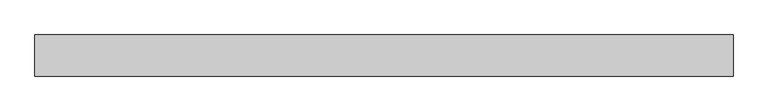
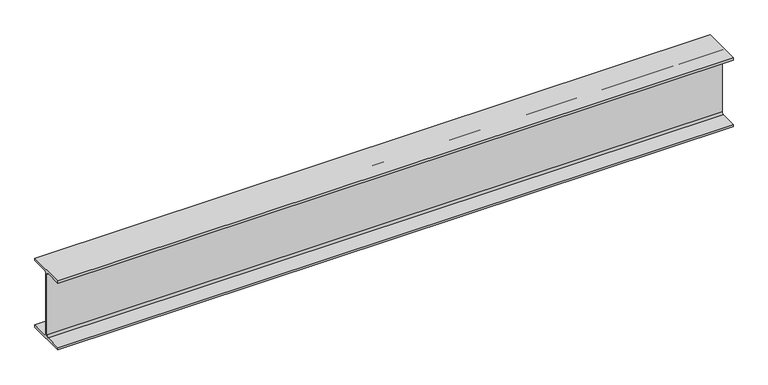
"""IFC4 building model written with IfcOpenShell, lengths in millimetres: beam geometry, Steel Beam_H-KSD3502 : H_SB_ASB_H-200x200x8x12."""

import ifcopenshell
import ifcopenshell.guid

model = None  # the IFC model being written
_history = None  # IfcOwnerHistory: only IFC2X3 demands one
_inside = {}  # id of a spatial element -> (the spatial element, [elements in it])
_under = {}  # id of a project, library or spatial element -> (it, [spatial elements below it])
_declared = {}  # id of a project -> (the project, [libraries it declares])
_typed = {}  # id of a type object -> (the type object, [elements of that type])
_made_of = {}  # id of a material, layer set ... -> (it, [elements and type objects made of it])


def new_model(schema):
    """Start an empty IFC model of exactly this schema.

    Asked for "IFC4X3", IfcOpenShell would pick the latest addendum, in which some entities
    have other attributes; the version numbers below select the first issue.
    IFC2X3 requires an IfcOwnerHistory on every rooted entity: one is made here for all.
    """
    global model, _history
    if schema == "IFC4X3":
        model = ifcopenshell.file(schema_version=(4, 3, 0, 0))
    else:
        model = ifcopenshell.file(schema=schema)
    _inside.clear()
    _under.clear()
    _declared.clear()
    _typed.clear()
    _made_of.clear()
    _history = None
    if model.schema == "IFC2X3":
        org = make("IfcOrganization", Name="unknown")
        user = make(
            "IfcPersonAndOrganization",
            ThePerson=make("IfcPerson", FamilyName="unknown"),
            TheOrganization=org,
        )
        app = make(
            "IfcApplication",
            ApplicationDeveloper=org,
            Version="unknown",
            ApplicationFullName="unknown",
            ApplicationIdentifier="unknown",
        )
        _history = make(
            "IfcOwnerHistory",
            OwningUser=user,
            OwningApplication=app,
            ChangeAction="ADDED",
            CreationDate=0,
        )
    return model


def make(cls, **values):
    """One entity of the class cls with the attributes given. An attribute that is None is left unset."""
    return model.create_entity(
        cls, **{name: value for name, value in values.items() if value is not None}
    )


def rooted(cls, **values):
    """An entity with a GlobalId (a new one), such as an element, a storey or a relation."""
    return make(cls, GlobalId=ifcopenshell.guid.new(), OwnerHistory=_history, **values)


def si_unit(unit_type, name, prefix=None):
    """IfcSIUnit, for example si_unit("LENGTHUNIT", "METRE", prefix="MILLI")."""
    return make("IfcSIUnit", UnitType=unit_type, Prefix=prefix, Name=name)


def assignment(units):
    """IfcUnitAssignment: the units of a project."""
    return None if units is None else make("IfcUnitAssignment", Units=units)


def point(xyz):
    """IfcCartesianPoint."""
    return None if xyz is None else make("IfcCartesianPoint", Coordinates=xyz)


def direction(xyz):
    """IfcDirection."""
    return None if xyz is None else make("IfcDirection", DirectionRatios=xyz)


def frame(location, z_axis=None, x_axis=None):
    """IfcAxis2Placement3D, a coordinate frame: its origin and axes. An axis left out is left unset."""
    return make(
        "IfcAxis2Placement3D",
        Location=point(location),
        Axis=direction(z_axis),
        RefDirection=direction(x_axis),
    )


def frame_2d(location, x_axis=None):
    """IfcAxis2Placement2D, a coordinate frame in the plane: its origin and x axis."""
    return make(
        "IfcAxis2Placement2D", Location=point(location), RefDirection=direction(x_axis)
    )


def origin():
    """The frame at (0, 0, 0) with its axes left unset."""
    return frame((0.0, 0.0, 0.0))


def place(relative_to, where):
    """IfcLocalPlacement: puts the frame where relative to a parent placement (None: the world)."""
    return make(
        "IfcLocalPlacement", PlacementRelTo=relative_to, RelativePlacement=where
    )


def context(
    kind, dimensions, precision=None, world=None, true_north=None, identifier=None
):
    """IfcGeometricRepresentationContext, for example the 3D "Model" context."""
    return make(
        "IfcGeometricRepresentationContext",
        ContextIdentifier=identifier,
        ContextType=kind,
        CoordinateSpaceDimension=dimensions,
        Precision=precision,
        WorldCoordinateSystem=world,
        TrueNorth=true_north,
    )


def project(units=None, contexts=None):
    """IfcProject with its units and contexts."""
    return rooted(
        "IfcProject",
        Name="project",
        RepresentationContexts=contexts,
        UnitsInContext=assignment(units),
    )


def spatial(cls, under=None, at=None, **own):
    """A site, building, storey or space (cls), placed at a placement, below another one or the project."""
    s = rooted(cls, ObjectPlacement=at, **own)
    if under is not None:
        _under.setdefault(under.id(), (under, []))[1].append(s)
    return s


def polyline(points):
    """IfcPolyline through the points."""
    return make("IfcPolyline", Points=[point(p) for p in points])


def circle_curve(where, radius):
    """IfcCircle in the frame where."""
    return make("IfcCircle", Position=where, Radius=radius)


def trimmed(basis, trim1, trim2, sense, master):
    """IfcTrimmedCurve: the piece of a basis curve between two trims."""
    return make(
        "IfcTrimmedCurve",
        BasisCurve=basis,
        Trim1=trim1,
        Trim2=trim2,
        SenseAgreement=sense,
        MasterRepresentation=master,
    )


def segment(curve, same_sense, transition):
    """IfcCompositeCurveSegment."""
    return make(
        "IfcCompositeCurveSegment",
        Transition=transition,
        SameSense=same_sense,
        ParentCurve=curve,
    )


def composite_curve(segments, self_intersect=None):
    """IfcCompositeCurve: segments joined end to end."""
    return make("IfcCompositeCurve", Segments=segments, SelfIntersect=self_intersect)


def outline(outer, holes=None, kind="AREA"):
    """IfcArbitraryClosedProfileDef: a profile drawn as a closed curve; with holes, ...WithVoids."""
    if holes is None:
        return make("IfcArbitraryClosedProfileDef", ProfileType=kind, OuterCurve=outer)
    return make(
        "IfcArbitraryProfileDefWithVoids",
        ProfileType=kind,
        OuterCurve=outer,
        InnerCurves=holes,
    )


def extrude(swept, where, along, depth):
    """IfcExtrudedAreaSolid: the profile swept, set in the frame where, extruded along a direction by depth."""
    return make(
        "IfcExtrudedAreaSolid",
        SweptArea=swept,
        Position=where,
        ExtrudedDirection=direction(along),
        Depth=depth,
    )


def shape(context_of_items, identifier, shape_type, items):
    """IfcShapeRepresentation: the items that make up one representation, for example the "Body"."""
    return make(
        "IfcShapeRepresentation",
        ContextOfItems=context_of_items,
        RepresentationIdentifier=identifier,
        RepresentationType=shape_type,
        Items=items,
    )


def source(mapping_origin, context_of_items, identifier, shape_type, items):
    """IfcRepresentationMap: a shape defined once, which mapped items show again and again."""
    return make(
        "IfcRepresentationMap",
        MappingOrigin=mapping_origin,
        MappedRepresentation=shape(context_of_items, identifier, shape_type, items),
    )


def transform(
    local_origin,
    x_axis=None,
    y_axis=None,
    z_axis=None,
    scale=None,
    scale2=None,
    scale3=None,
    uniform=True,
):
    """IfcCartesianTransformationOperator3D, or its non-uniform kind. x_axis, y_axis, z_axis: its Axis1, 2, 3."""
    if uniform:
        return make(
            "IfcCartesianTransformationOperator3D",
            Axis1=direction(x_axis),
            Axis2=direction(y_axis),
            LocalOrigin=point(local_origin),
            Scale=scale,
            Axis3=direction(z_axis),
        )
    return make(
        "IfcCartesianTransformationOperator3DnonUniform",
        Axis1=direction(x_axis),
        Axis2=direction(y_axis),
        LocalOrigin=point(local_origin),
        Scale=scale,
        Axis3=direction(z_axis),
        Scale2=scale2,
        Scale3=scale3,
    )


def mapped(mapping_source, mapping_target):
    """IfcMappedItem: shows the shape of a source again, moved by a transform."""
    return make(
        "IfcMappedItem", MappingSource=mapping_source, MappingTarget=mapping_target
    )


def made_of(thing, what):
    """Note that an element or type object is made of a material, layer set ...; save() writes the relation."""
    if what is not None:
        _made_of.setdefault(what.id(), (what, []))[1].append(thing)
    return thing


def element(
    cls,
    number,
    at=None,
    inside=None,
    cuts=None,
    type_object=None,
    material=None,
    context=None,
    identifier="Body",
    shape_type=None,
    held_by="IfcProductDefinitionShape",
    body=None,
    shapes=None,
    **own,
):
    """One element of the class cls, such as IfcWall. Its Tag is "e" and its number.

    at: its placement. inside: the storey or other place that contains it. cuts: it is an
    opening in that element (IfcRelVoidsElement). A single representation is given by context,
    identifier, shape_type and body (its items); several are given by shapes. held_by: the class
    of the entity that holds the representations. save() writes the other relations.
    """
    e = rooted(cls, Tag="e%d" % number, ObjectPlacement=at, **own)
    if body is not None:
        shapes = [shape(context, identifier, shape_type, body)]
    if shapes is not None:
        e.Representation = make(held_by, Representations=shapes)
    if inside is not None:
        _inside.setdefault(inside.id(), (inside, []))[1].append(e)
    if cuts is not None:
        rooted(
            "IfcRelVoidsElement", RelatingBuildingElement=cuts, RelatedOpeningElement=e
        )
    if type_object is not None:
        _typed.setdefault(type_object.id(), (type_object, []))[1].append(e)
    return made_of(e, material)


def aggregate(whole, parts):
    """IfcRelAggregates: a whole, such as a stair, and the parts it consists of."""
    return rooted("IfcRelAggregates", RelatingObject=whole, RelatedObjects=parts)


def save(model, path):
    """Write the relations noted so far, then the file.

    IfcRelAggregates (storeys below a building ...), IfcRelContainedInSpatialStructure (elements
    in a storey), IfcRelDefinesByType, IfcRelAssociatesMaterial and IfcRelDeclares: one each for
    every whole, place, type object, material and project.
    """
    for whole, parts in _under.values():
        aggregate(whole, parts)
    for where, things in _inside.values():
        rooted(
            "IfcRelContainedInSpatialStructure",
            RelatedElements=things,
            RelatingStructure=where,
        )
    for kind, things in _typed.values():
        rooted("IfcRelDefinesByType", RelatedObjects=things, RelatingType=kind)
    for what, things in _made_of.values():
        rooted("IfcRelAssociatesMaterial", RelatedObjects=things, RelatingMaterial=what)
    for by, libraries in _declared.values():
        rooted("IfcRelDeclares", RelatingContext=by, RelatedDefinitions=libraries)
    model.write(path)


def beam_da187b0d(model_context):
    return source(origin(), model_context, "Body", "SweptSolid", [
        extrude(outline(composite_curve([segment(polyline([(82.5, -141.5), (82.5, -151.7), (-82.5, -151.7), (-82.5, -141.5), (-11.9, -141.5)]), True, "CONTINUOUS"), segment(trimmed(circle_curve(frame_2d((-11.9, -132.6)), 8.9), [point((-11.9, -141.5))], [point((-3.0, -132.6))], True, "CARTESIAN"), True, "CONTINUOUS"), segment(polyline([(-3.0, -132.6), (-3.0, 132.6)]), True, "CONTINUOUS"), segment(trimmed(circle_curve(frame_2d((-11.9, 132.6)), 8.9), [point((-3.0, 132.6))], [point((-11.9, 141.5))], True, "CARTESIAN"), True, "CONTINUOUS"), segment(polyline([(-11.9, 141.5), (-82.5, 141.5), (-82.5, 151.7), (82.5, 151.7), (82.5, 141.5), (11.9, 141.5)]), True, "CONTINUOUS"), segment(trimmed(circle_curve(frame_2d((11.9, 132.6)), 8.9), [point((11.9, 141.5))], [point((3.0, 132.6))], True, "CARTESIAN"), True, "CONTINUOUS"), segment(polyline([(3.0, 132.6), (3.0, -132.6)]), True, "CONTINUOUS"), segment(trimmed(circle_curve(frame_2d((11.9, -132.6)), 8.9), [point((3.0, -132.6))], [point((11.9, -141.5))], True, "CARTESIAN"), True, "CONTINUOUS"), segment(polyline([(11.9, -141.5), (82.5, -141.5)]), True, "CONTINUOUS")], self_intersect=False)), frame((-1369.9070509, 0.0, 0.0), z_axis=(1.0, 0.0, 0.0), x_axis=(0.0, 1.0, 0.0)), (0.0, 0.0, 1.0), 2801.3094314),
    ])


if __name__ == "__main__":
    model = new_model("IFC4")
    model_context = context("Model", 3, world=origin())
    ifc_project = project(units=[si_unit("LENGTHUNIT", "METRE", prefix="MILLI")], contexts=[model_context])
    site = spatial("IfcSite", under=ifc_project)
    building = spatial("IfcBuilding", under=site)
    placement = place(None, origin())
    beam_shape = beam_da187b0d(model_context)
    element("IfcBeam", 1, ObjectType="Steel Beam_H-KSD3502 : H_SB_ASB_H-200x200x8x12", at=placement, inside=building, context=model_context, shape_type="MappedRepresentation", body=[
        mapped(beam_shape, transform((0.0, 0.0, 0.0), x_axis=(1.0, 0.0, 0.0), y_axis=(0.0, 1.0, 0.0), z_axis=(0.0, 0.0, 1.0))),
    ])
    save(model, "model.ifc")

# Revit data of these elements
# Type "Steel Beam_H-KSD3502 : H_SB_ASB_H-200x200x8x12"
#   Width = 20.0 cm
#   Web Thickness = 0.8 cm
#   Web Fillet = 1.3 cm
#   Warping Constant = 141376.0 cm⁶
#   Torsional Moment of Inertia = 26.2485 cm⁴
#   Torsional Modulus = 1.0 cm³
#   Section Area = 63.53 cm²
#   Plastic Modulus weak axis = 244.0 cm³
#   Plastic Modulus strong axis = 525.0 cm³
#   Perimeter = 1.16 m²/m
#   Nominal Weight = 49.90 kgf/m
#   Moment of Inertia weak axis = 1600.00 cm⁴
#   Moment of Inertia strong axis = 4720.00 cm⁴
#   Height = 20.0 cm
#   Flange Thickness = 1.2 cm
#   Elastic Modulus weak axis = 160.0 cm³
#   Elastic Modulus strong axis = 472.0 cm³
#   Centroid Vertical = 10.0 cm
#   Centroid Horizontal = 10.0 cm
#   Length [instance default] = 1.5240 m
#   Structural Material [instance default] = Steel, 45-345
#   Assembly Code = ""
# Element 1 (IfcBeam, "Steel Beam_H-KSD3502 : H_SB_ASB_H-200x200x8x12")
#   Structural Material = none
# Materials
#   "Steel, 45-345": class "Metal", colour RGB 189 187 185, transparency 0, Description = "Steel 345 MPa", Cost = 0
